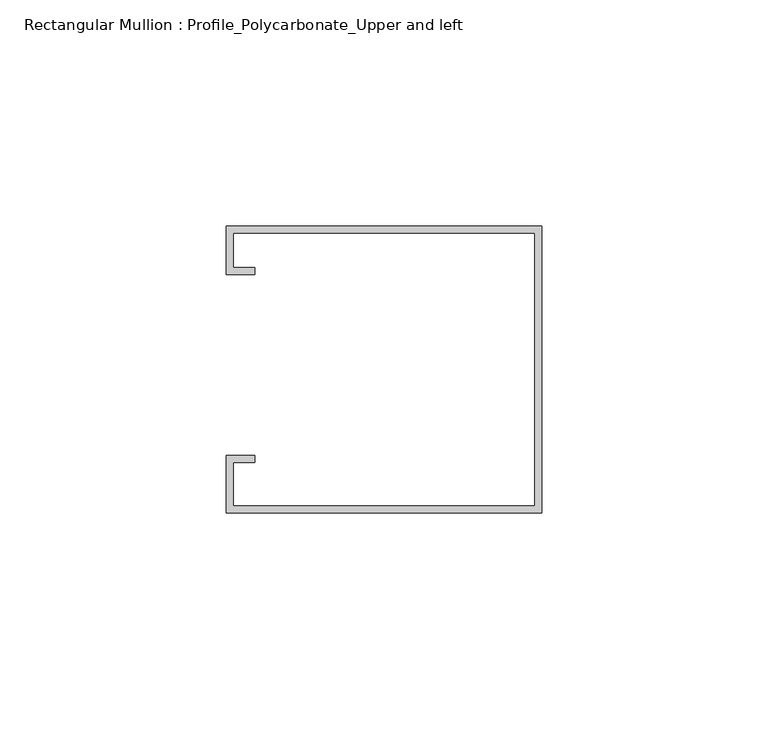
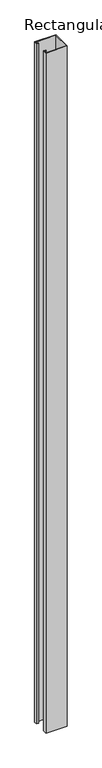
"""IFC4 building model written with IfcOpenShell, lengths in millimetres: member geometry, Rectangular Mullion : Profile_Polycarbonate_Upper and left."""

from ifc_helpers import new_model, si_unit, frame, origin, place, context, project, spatial, polyline, outline, extrude, source, transform, mapped, element, save


def rectangular_mullion_profile_polycarbonate_upper_and_left_498f4f23(model_context):
    return source(origin(), model_context, "Body", "SweptSolid", [
        extrude(outline(polyline([(0.0, -32.7), (-69.85, -32.7), (-69.85, -20.0), (-63.5, -20.0), (-63.5, -21.5875), (-68.2625, -21.5875), (-68.2625, -31.1125), (-1.5875, -31.1125), (-1.5875, 29.2125), (-68.2625, 29.2125), (-68.2625, 21.5875), (-63.5, 21.5875), (-63.5, 20.0), (-69.85, 20.0), (-69.85, 30.8), (0.0, 30.8), (0.0, -32.7)])), frame((0.0, 0.0, -2362.2), z_axis=(0.0, 0.0, 1.0), x_axis=(1.0, 0.0, 0.0)), (0.0, 0.0, 1.0), 2362.2),
    ])


if __name__ == "__main__":
    model = new_model("IFC4")
    model_context = context("Model", 3, world=origin())
    ifc_project = project(units=[si_unit("LENGTHUNIT", "METRE", prefix="MILLI")], contexts=[model_context])
    site = spatial("IfcSite", under=ifc_project)
    building = spatial("IfcBuilding", under=site)
    placement = place(None, origin())
    rectangular_mullion_profile_polycarbonate_upper_and_left_shape = rectangular_mullion_profile_polycarbonate_upper_and_left_498f4f23(model_context)
    element("IfcMember", 1, ObjectType="Rectangular Mullion : Profile_Polycarbonate_Upper and left", at=placement, inside=building, context=model_context, shape_type="MappedRepresentation", body=[
        mapped(rectangular_mullion_profile_polycarbonate_upper_and_left_shape, transform((0.0, 0.0, 0.0), x_axis=(1.0, 0.0, 0.0), y_axis=(0.0, 1.0, 0.0), z_axis=(0.0, 0.0, 1.0))),
    ])
    save(model, "model.ifc")

# Revit data of these elements
# Type "Rectangular Mullion : Profile_Polycarbonate_Upper and left"
#   built-in parameter 1007322 = 0.208333 (stored number, unit not read)
#   built-in parameter 1007321 = 0.00520833 (stored number, unit not read)
#   built-in parameter 1007320 = 0 (stored number, unit not read)
# Element 1 (IfcMember, "Rectangular Mullion : Profile_Polycarbonate_Upper and left")
#   Materials on its faces: "ALUMINUM PROFILE AT POLYCARBONATE PANEL"
# Materials
#   "ALUMINUM PROFILE AT POLYCARBONATE PANEL": class "Metal", colour RGB 244 244 244, transparency 0, Description = "Aluminum 6061", Cost = 0
